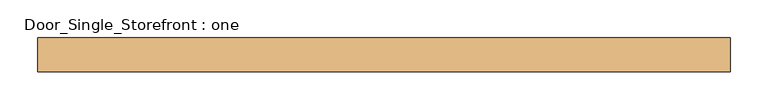
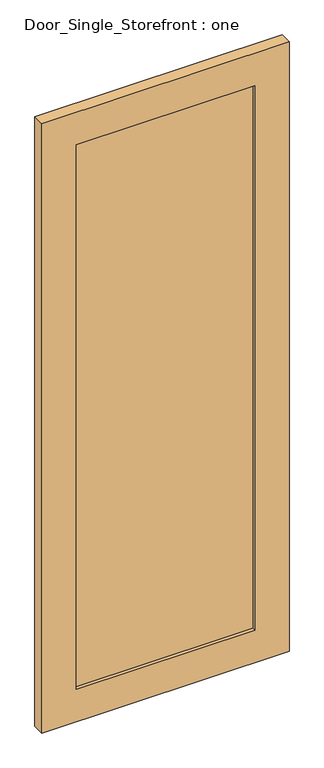
"""IFC4 building model written with IfcOpenShell, lengths in millimetres: door geometry, Door_Single_Storefront : one."""

from ifc_helpers import new_model, si_unit, frame, origin, place, context, project, spatial, polyline, outline, extrude, source, transform, mapped, element, save


def door_single_storefront_one_9ede4525(model_context):
    return source(origin(), model_context, "Body", "SweptSolid", [
        extrude(outline(polyline([(330.2, -6.35), (-330.2, -6.35), (-330.2, 12.7), (330.2, 12.7), (330.2, -6.35)])), frame((0.0, 0.0, 127.0), z_axis=(0.0, 0.0, 1.0), x_axis=(1.0, 0.0, 0.0)), (0.0, 0.0, 1.0), 2129.5688887),
        extrude(outline(polyline([(2383.5688887, -457.2), (0.0, -457.2), (0.0, 457.2), (2383.5688887, 457.2), (2383.5688887, -457.2)]), holes=[polyline([(127.0, 330.2), (127.0, -330.2), (2256.5688887, -330.2), (2256.5688887, 330.2), (127.0, 330.2)])]), frame((0.0, -19.05, 0.0), z_axis=(0.0, 1.0, 0.0), x_axis=(0.0, 0.0, 1.0)), (0.0, 0.0, 1.0), 44.45),
    ])


if __name__ == "__main__":
    model = new_model("IFC4")
    model_context = context("Model", 3, world=origin())
    ifc_project = project(units=[si_unit("LENGTHUNIT", "METRE", prefix="MILLI")], contexts=[model_context])
    site = spatial("IfcSite", under=ifc_project)
    building = spatial("IfcBuilding", under=site)
    placement = place(None, origin())
    door_single_storefront_one_shape = door_single_storefront_one_9ede4525(model_context)
    element("IfcDoor", 1, ObjectType="Door_Single_Storefront : one", at=placement, inside=building, context=model_context, shape_type="MappedRepresentation", body=[
        mapped(door_single_storefront_one_shape, transform((0.0, 0.0, 0.0), x_axis=(1.0, 0.0, 0.0), y_axis=(0.0, 1.0, 0.0), z_axis=(0.0, 0.0, 1.0))),
    ])
    save(model, "model.ifc")

# Revit data of these elements
# Type "Door_Single_Storefront : one"
#   Type Mark = "29"
#   Analytic Construction = "<None>"
#   Stile_Width = 0' - 5"
#   Door_Thickness = 0' - 1 3/4"
#   Door_Offset = 0' - 1"
#   Glass_Material = ALUM. STOREFRONT W/ INSULATED GLAZING
#   Frame_Material = Aluminum
#   Function = (empty or 0)
# Element 1 (IfcDoor, "Door_Single_Storefront : one")
#   Materials on its faces: "Aluminum", "ALUM. STOREFRONT W/ INSULATED GLAZING"
# Materials
#   "ALUM. STOREFRONT W/ INSULATED GLAZING": class "Glass", colour RGB 196 205 210, transparency 0.85, Description = "Soda Lime Glass", Cost = 0
#   "Aluminum": class "Metal", colour RGB 244 244 244, transparency 0, Description = "Aluminum 6061", Cost = 0
